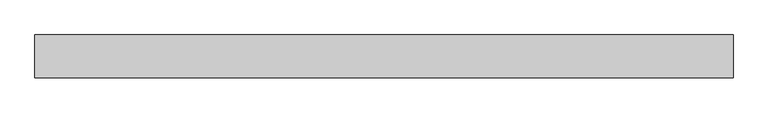
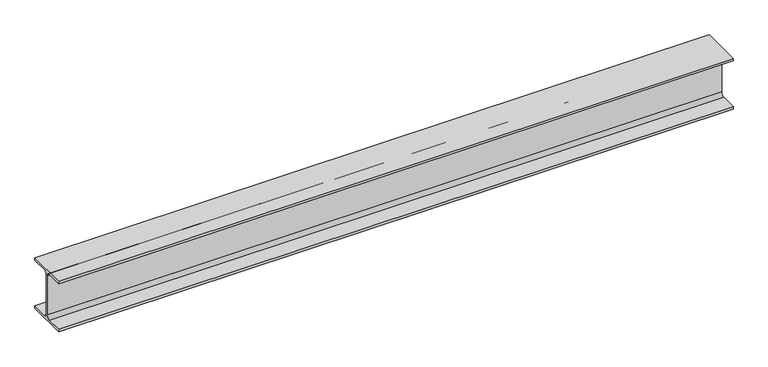
"""IFC4 building model written with IfcOpenShell, lengths in millimetres: beam geometry, 0912_Steel Framing_H-KSD3502 : H_SB_ASB_H-194x150x6x9."""

from ifc_helpers import new_model, si_unit, point, frame, frame_2d, origin, place, context, project, spatial, polyline, circle_curve, trimmed, segment, composite_curve, outline, extrude, source, transform, mapped, element, save


def beam_49090cc4(model_context):
    return source(origin(), model_context, "Body", "SweptSolid", [
        extrude(outline(composite_curve([segment(polyline([(75.0, -88.0), (75.0, -97.0), (-75.0, -97.0), (-75.0, -88.0), (-16.0, -88.0)]), True, "CONTINUOUS"), segment(trimmed(circle_curve(frame_2d((-16.0, -75.0)), 13.0), [point((-16.0, -88.0))], [point((-3.0, -75.0))], True, "CARTESIAN"), True, "CONTINUOUS"), segment(polyline([(-3.0, -75.0), (-3.0, 75.0)]), True, "CONTINUOUS"), segment(trimmed(circle_curve(frame_2d((-16.0, 75.0)), 13.0), [point((-3.0, 75.0))], [point((-16.0, 88.0))], True, "CARTESIAN"), True, "CONTINUOUS"), segment(polyline([(-16.0, 88.0), (-75.0, 88.0), (-75.0, 97.0), (75.0, 97.0), (75.0, 88.0), (16.0, 88.0)]), True, "CONTINUOUS"), segment(trimmed(circle_curve(frame_2d((16.0, 75.0)), 13.0), [point((16.0, 88.0))], [point((3.0, 75.0))], True, "CARTESIAN"), True, "CONTINUOUS"), segment(polyline([(3.0, 75.0), (3.0, -75.0)]), True, "CONTINUOUS"), segment(trimmed(circle_curve(frame_2d((16.0, -75.0)), 13.0), [point((3.0, -75.0))], [point((16.0, -88.0))], True, "CARTESIAN"), True, "CONTINUOUS"), segment(polyline([(16.0, -88.0), (75.0, -88.0)]), True, "CONTINUOUS")], self_intersect=False)), frame((-1200.0, 0.0, 0.0), z_axis=(1.0, 0.0, 0.0), x_axis=(0.0, 1.0, 0.0)), (0.0, 0.0, 1.0), 2453.1701073),
    ])


if __name__ == "__main__":
    model = new_model("IFC4")
    model_context = context("Model", 3, world=origin())
    ifc_project = project(units=[si_unit("LENGTHUNIT", "METRE", prefix="MILLI")], contexts=[model_context])
    site = spatial("IfcSite", under=ifc_project)
    building = spatial("IfcBuilding", under=site)
    placement = place(None, origin())
    beam_shape = beam_49090cc4(model_context)
    element("IfcBeam", 1, ObjectType="0912_Steel Framing_H-KSD3502 : H_SB_ASB_H-194x150x6x9", at=placement, inside=building, context=model_context, shape_type="MappedRepresentation", body=[
        mapped(beam_shape, transform((0.0, 0.0, 0.0), x_axis=(1.0, 0.0, 0.0), y_axis=(0.0, 1.0, 0.0), z_axis=(0.0, 0.0, 1.0))),
    ])
    save(model, "model.ifc")

# Revit data of these elements
# Type "0912_Steel Framing_H-KSD3502 : H_SB_ASB_H-194x150x6x9"
#   H_WM Code_1 = "S01AA002-00001 | Main Steel Structure Fabrication Work | Shelter/Building | Medium Steel - Standard (90KG/M>Weight≥30KG/M) | Material: (   )"
#   H_WM Code_2 = "S03AA028-00001 | Main Steel Structure Erection Work | Shelter/Building | Medium Steel (90KG/M>Weight≥30KG/M) | Material: (   )"
#   H_WM Code_3 = "S01AA010-00001 | Main Steel Structure Fabrication Work | Shelter/Building | Steel Painting/Coating | for Non-Fireproofed Steel Surface, Surface Preparation, Primer, Second & Final Coat | Material: (   )"
#   H_Q'ty Cal Type Tag = "SB-Q2"
#   Width = 15.0 cm
#   Web Thickness = 0.6 cm
#   Web Fillet = 1.3 cm
#   Warping Constant = 43316.0 cm⁶
#   W = 0
#   Torsional Moment of Inertia = 8.622 cm⁴
#   Section Area = 39.01 cm²
#   Plastic Modulus weak axis = 104.0 cm³
#   Plastic Modulus strong axis = 309.0 cm³
#   Perimeter = 0.95 m²/m
#   Nominal Weight = 30.60 kgf/m
#   Moment of Inertia weak axis = 507.00 cm⁴
#   Moment of Inertia strong axis = 2690.00 cm⁴
#   Height = 19.4 cm
#   Flange Thickness = 0.9 cm
#   Elastic Modulus weak axis = 67.6 cm³
#   Elastic Modulus strong axis = 277.0 cm³
#   Centroid Vertical = 9.7 cm
#   Centroid Horizontal = 7.5 cm
#   Ix = 26900000
#   Length [instance default] = 1.5240 m
#   Zx = 309000
#   b = 0.1500 m
#   h = 0.1940 m
#   r = 0.0130 m
#   s = 0.0060 m
#   t = 0.0090 m
#   A = 0.003901 m²
#   Structural Material [instance default] = Steel, 45-345
#   Assembly Code = ""
# Element 1 (IfcBeam, "0912_Steel Framing_H-KSD3502 : H_SB_ASB_H-194x150x6x9")
#   Structural Material = none
# Materials
#   "Steel, 45-345": class "Metal", colour RGB 189 187 185, transparency 0, Description = "Steel 345 MPa", Cost = 0
